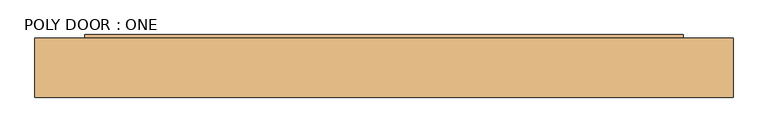
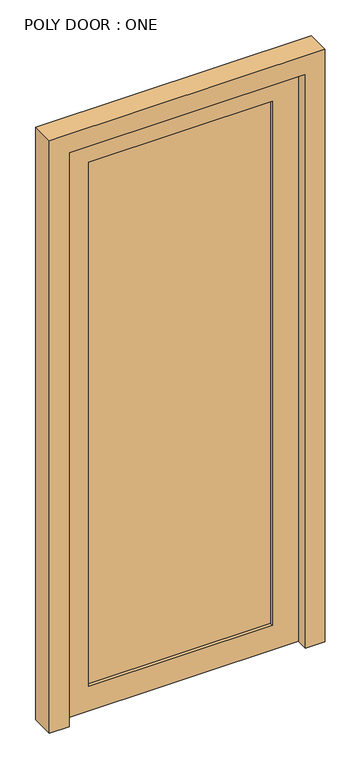
"""IFC4 building model written with IfcOpenShell, lengths in millimetres: door geometry, POLY DOOR : ONE."""

import ifcopenshell
import ifcopenshell.guid

model = None  # the IFC model being written
_history = None  # IfcOwnerHistory: only IFC2X3 demands one
_inside = {}  # id of a spatial element -> (the spatial element, [elements in it])
_under = {}  # id of a project, library or spatial element -> (it, [spatial elements below it])
_declared = {}  # id of a project -> (the project, [libraries it declares])
_typed = {}  # id of a type object -> (the type object, [elements of that type])
_made_of = {}  # id of a material, layer set ... -> (it, [elements and type objects made of it])


def new_model(schema):
    """Start an empty IFC model of exactly this schema.

    Asked for "IFC4X3", IfcOpenShell would pick the latest addendum, in which some entities
    have other attributes; the version numbers below select the first issue.
    IFC2X3 requires an IfcOwnerHistory on every rooted entity: one is made here for all.
    """
    global model, _history
    if schema == "IFC4X3":
        model = ifcopenshell.file(schema_version=(4, 3, 0, 0))
    else:
        model = ifcopenshell.file(schema=schema)
    _inside.clear()
    _under.clear()
    _declared.clear()
    _typed.clear()
    _made_of.clear()
    _history = None
    if model.schema == "IFC2X3":
        org = make("IfcOrganization", Name="unknown")
        user = make(
            "IfcPersonAndOrganization",
            ThePerson=make("IfcPerson", FamilyName="unknown"),
            TheOrganization=org,
        )
        app = make(
            "IfcApplication",
            ApplicationDeveloper=org,
            Version="unknown",
            ApplicationFullName="unknown",
            ApplicationIdentifier="unknown",
        )
        _history = make(
            "IfcOwnerHistory",
            OwningUser=user,
            OwningApplication=app,
            ChangeAction="ADDED",
            CreationDate=0,
        )
    return model


def make(cls, **values):
    """One entity of the class cls with the attributes given. An attribute that is None is left unset."""
    return model.create_entity(
        cls, **{name: value for name, value in values.items() if value is not None}
    )


def rooted(cls, **values):
    """An entity with a GlobalId (a new one), such as an element, a storey or a relation."""
    return make(cls, GlobalId=ifcopenshell.guid.new(), OwnerHistory=_history, **values)


def si_unit(unit_type, name, prefix=None):
    """IfcSIUnit, for example si_unit("LENGTHUNIT", "METRE", prefix="MILLI")."""
    return make("IfcSIUnit", UnitType=unit_type, Prefix=prefix, Name=name)


def assignment(units):
    """IfcUnitAssignment: the units of a project."""
    return None if units is None else make("IfcUnitAssignment", Units=units)


def point(xyz):
    """IfcCartesianPoint."""
    return None if xyz is None else make("IfcCartesianPoint", Coordinates=xyz)


def direction(xyz):
    """IfcDirection."""
    return None if xyz is None else make("IfcDirection", DirectionRatios=xyz)


def frame(location, z_axis=None, x_axis=None):
    """IfcAxis2Placement3D, a coordinate frame: its origin and axes. An axis left out is left unset."""
    return make(
        "IfcAxis2Placement3D",
        Location=point(location),
        Axis=direction(z_axis),
        RefDirection=direction(x_axis),
    )


def origin():
    """The frame at (0, 0, 0) with its axes left unset."""
    return frame((0.0, 0.0, 0.0))


def place(relative_to, where):
    """IfcLocalPlacement: puts the frame where relative to a parent placement (None: the world)."""
    return make(
        "IfcLocalPlacement", PlacementRelTo=relative_to, RelativePlacement=where
    )


def context(
    kind, dimensions, precision=None, world=None, true_north=None, identifier=None
):
    """IfcGeometricRepresentationContext, for example the 3D "Model" context."""
    return make(
        "IfcGeometricRepresentationContext",
        ContextIdentifier=identifier,
        ContextType=kind,
        CoordinateSpaceDimension=dimensions,
        Precision=precision,
        WorldCoordinateSystem=world,
        TrueNorth=true_north,
    )


def project(units=None, contexts=None):
    """IfcProject with its units and contexts."""
    return rooted(
        "IfcProject",
        Name="project",
        RepresentationContexts=contexts,
        UnitsInContext=assignment(units),
    )


def spatial(cls, under=None, at=None, **own):
    """A site, building, storey or space (cls), placed at a placement, below another one or the project."""
    s = rooted(cls, ObjectPlacement=at, **own)
    if under is not None:
        _under.setdefault(under.id(), (under, []))[1].append(s)
    return s


def polyline(points):
    """IfcPolyline through the points."""
    return make("IfcPolyline", Points=[point(p) for p in points])


def outline(outer, holes=None, kind="AREA"):
    """IfcArbitraryClosedProfileDef: a profile drawn as a closed curve; with holes, ...WithVoids."""
    if holes is None:
        return make("IfcArbitraryClosedProfileDef", ProfileType=kind, OuterCurve=outer)
    return make(
        "IfcArbitraryProfileDefWithVoids",
        ProfileType=kind,
        OuterCurve=outer,
        InnerCurves=holes,
    )


def extrude(swept, where, along, depth):
    """IfcExtrudedAreaSolid: the profile swept, set in the frame where, extruded along a direction by depth."""
    return make(
        "IfcExtrudedAreaSolid",
        SweptArea=swept,
        Position=where,
        ExtrudedDirection=direction(along),
        Depth=depth,
    )


def shape(context_of_items, identifier, shape_type, items):
    """IfcShapeRepresentation: the items that make up one representation, for example the "Body"."""
    return make(
        "IfcShapeRepresentation",
        ContextOfItems=context_of_items,
        RepresentationIdentifier=identifier,
        RepresentationType=shape_type,
        Items=items,
    )


def source(mapping_origin, context_of_items, identifier, shape_type, items):
    """IfcRepresentationMap: a shape defined once, which mapped items show again and again."""
    return make(
        "IfcRepresentationMap",
        MappingOrigin=mapping_origin,
        MappedRepresentation=shape(context_of_items, identifier, shape_type, items),
    )


def transform(
    local_origin,
    x_axis=None,
    y_axis=None,
    z_axis=None,
    scale=None,
    scale2=None,
    scale3=None,
    uniform=True,
):
    """IfcCartesianTransformationOperator3D, or its non-uniform kind. x_axis, y_axis, z_axis: its Axis1, 2, 3."""
    if uniform:
        return make(
            "IfcCartesianTransformationOperator3D",
            Axis1=direction(x_axis),
            Axis2=direction(y_axis),
            LocalOrigin=point(local_origin),
            Scale=scale,
            Axis3=direction(z_axis),
        )
    return make(
        "IfcCartesianTransformationOperator3DnonUniform",
        Axis1=direction(x_axis),
        Axis2=direction(y_axis),
        LocalOrigin=point(local_origin),
        Scale=scale,
        Axis3=direction(z_axis),
        Scale2=scale2,
        Scale3=scale3,
    )


def mapped(mapping_source, mapping_target):
    """IfcMappedItem: shows the shape of a source again, moved by a transform."""
    return make(
        "IfcMappedItem", MappingSource=mapping_source, MappingTarget=mapping_target
    )


def made_of(thing, what):
    """Note that an element or type object is made of a material, layer set ...; save() writes the relation."""
    if what is not None:
        _made_of.setdefault(what.id(), (what, []))[1].append(thing)
    return thing


def element(
    cls,
    number,
    at=None,
    inside=None,
    cuts=None,
    type_object=None,
    material=None,
    context=None,
    identifier="Body",
    shape_type=None,
    held_by="IfcProductDefinitionShape",
    body=None,
    shapes=None,
    **own,
):
    """One element of the class cls, such as IfcWall. Its Tag is "e" and its number.

    at: its placement. inside: the storey or other place that contains it. cuts: it is an
    opening in that element (IfcRelVoidsElement). A single representation is given by context,
    identifier, shape_type and body (its items); several are given by shapes. held_by: the class
    of the entity that holds the representations. save() writes the other relations.
    """
    e = rooted(cls, Tag="e%d" % number, ObjectPlacement=at, **own)
    if body is not None:
        shapes = [shape(context, identifier, shape_type, body)]
    if shapes is not None:
        e.Representation = make(held_by, Representations=shapes)
    if inside is not None:
        _inside.setdefault(inside.id(), (inside, []))[1].append(e)
    if cuts is not None:
        rooted(
            "IfcRelVoidsElement", RelatingBuildingElement=cuts, RelatedOpeningElement=e
        )
    if type_object is not None:
        _typed.setdefault(type_object.id(), (type_object, []))[1].append(e)
    return made_of(e, material)


def aggregate(whole, parts):
    """IfcRelAggregates: a whole, such as a stair, and the parts it consists of."""
    return rooted("IfcRelAggregates", RelatingObject=whole, RelatedObjects=parts)


def save(model, path):
    """Write the relations noted so far, then the file.

    IfcRelAggregates (storeys below a building ...), IfcRelContainedInSpatialStructure (elements
    in a storey), IfcRelDefinesByType, IfcRelAssociatesMaterial and IfcRelDeclares: one each for
    every whole, place, type object, material and project.
    """
    for whole, parts in _under.values():
        aggregate(whole, parts)
    for where, things in _inside.values():
        rooted(
            "IfcRelContainedInSpatialStructure",
            RelatedElements=things,
            RelatingStructure=where,
        )
    for kind, things in _typed.values():
        rooted("IfcRelDefinesByType", RelatedObjects=things, RelatingType=kind)
    for what, things in _made_of.values():
        rooted("IfcRelAssociatesMaterial", RelatedObjects=things, RelatingMaterial=what)
    for by, libraries in _declared.values():
        rooted("IfcRelDeclares", RelatingContext=by, RelatedDefinitions=libraries)
    model.write(path)


def poly_door_one_c9e5c697(model_context):
    return source(origin(), model_context, "Body", "SweptSolid", [
        extrude(outline(polyline([(355.6, 25.4), (355.6, 12.7), (-355.6, 12.7), (-355.6, 25.4), (355.6, 25.4)])), frame((0.0, 0.0, 101.6), z_axis=(0.0, 0.0, 1.0), x_axis=(1.0, 0.0, 0.0)), (0.0, 0.0, 1.0), 2139.95),
        extrude(outline(polyline([(2343.15, 457.2), (2343.15, -457.2), (0.0, -457.2), (0.0, 457.2), (2343.15, 457.2)]), holes=[polyline([(2241.55, 355.6), (101.6, 355.6), (101.6, -355.6), (2241.55, -355.6), (2241.55, 355.6)])]), frame((0.0, 0.0, 0.0), z_axis=(0.0, 1.0, 0.0), x_axis=(0.0, 0.0, 1.0)), (0.0, 0.0, 1.0), 50.8),
        extrude(outline(polyline([(2419.35, -533.4), (0.0, -533.4), (0.0, -457.2), (2343.15, -457.2), (2343.15, 457.2), (0.0, 457.2), (0.0, 533.4), (2419.35, 533.4), (2419.35, -533.4)])), frame((0.0, -45.39996, 0.0), z_axis=(0.0, 1.0, 0.0), x_axis=(0.0, 0.0, 1.0)), (0.0, 0.0, 1.0), 90.79992),
    ])


if __name__ == "__main__":
    model = new_model("IFC4")
    model_context = context("Model", 3, world=origin())
    ifc_project = project(units=[si_unit("LENGTHUNIT", "METRE", prefix="MILLI")], contexts=[model_context])
    site = spatial("IfcSite", under=ifc_project)
    building = spatial("IfcBuilding", under=site)
    placement = place(None, origin())
    poly_door_one_shape = poly_door_one_c9e5c697(model_context)
    element("IfcDoor", 1, ObjectType="POLY DOOR : ONE", at=placement, inside=building, context=model_context, shape_type="MappedRepresentation", body=[
        mapped(poly_door_one_shape, transform((0.0, 0.0, 0.0), x_axis=(1.0, 0.0, 0.0), y_axis=(0.0, 1.0, 0.0), z_axis=(0.0, 0.0, 1.0))),
    ])
    save(model, "model.ifc")

# Revit data of these elements
# Type "POLY DOOR : ONE"
#   Type Mark = "53"
#   Assembly Code = "C1020"
#   Analytic Construction = "<None>"
#   Thickness = 0' - 2"
#   Glass Inset = 0' - 4"
#   Height = 7' - 8 1/4"
#   Trim Projection Ext = 0' - 1"
#   Trim Projection Int = 0' - 1"
#   Trim Width = 0' - 3"
#   Width = 3' - 0"
#   WINDOW = yes
#   Glass Material = ALUM. STOREFRONT W/ INSULATED GLAZING
#   Door Material = Aluminum
#   Frame Material = Aluminum
#   Function = (empty or 0)
#   Wall Closure = (empty or 0)
# Element 1 (IfcDoor, "POLY DOOR : ONE")
#   Materials on its faces: "Aluminum", "ALUM. STOREFRONT W/ INSULATED GLAZING"
# Materials
#   "ALUM. STOREFRONT W/ INSULATED GLAZING": class "Glass", colour RGB 196 205 210, transparency 0.85, Description = "Soda Lime Glass", Cost = 0
#   "Aluminum": class "Metal", colour RGB 244 244 244, transparency 0, Description = "Aluminum 6061", Cost = 0
